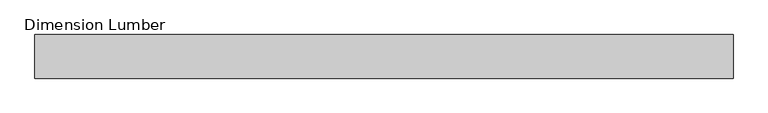
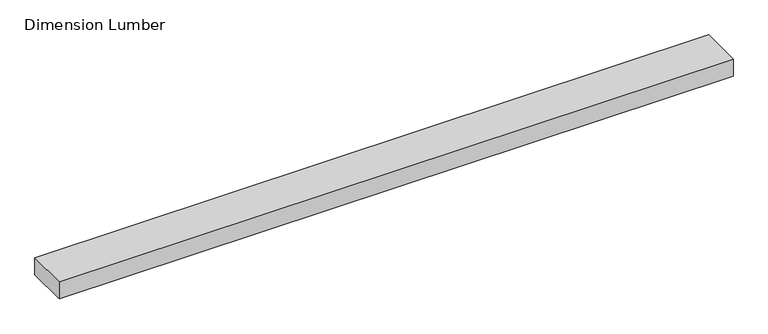
"""IFC4 building model written with IfcOpenShell, lengths in millimetres: beam geometry, Dimension Lumber : Top Supporting Lumbers."""

import ifcopenshell
import ifcopenshell.guid

model = None  # the IFC model being written
_history = None  # IfcOwnerHistory: only IFC2X3 demands one
_inside = {}  # id of a spatial element -> (the spatial element, [elements in it])
_under = {}  # id of a project, library or spatial element -> (it, [spatial elements below it])
_declared = {}  # id of a project -> (the project, [libraries it declares])
_typed = {}  # id of a type object -> (the type object, [elements of that type])
_made_of = {}  # id of a material, layer set ... -> (it, [elements and type objects made of it])


def new_model(schema):
    """Start an empty IFC model of exactly this schema.

    Asked for "IFC4X3", IfcOpenShell would pick the latest addendum, in which some entities
    have other attributes; the version numbers below select the first issue.
    IFC2X3 requires an IfcOwnerHistory on every rooted entity: one is made here for all.
    """
    global model, _history
    if schema == "IFC4X3":
        model = ifcopenshell.file(schema_version=(4, 3, 0, 0))
    else:
        model = ifcopenshell.file(schema=schema)
    _inside.clear()
    _under.clear()
    _declared.clear()
    _typed.clear()
    _made_of.clear()
    _history = None
    if model.schema == "IFC2X3":
        org = make("IfcOrganization", Name="unknown")
        user = make(
            "IfcPersonAndOrganization",
            ThePerson=make("IfcPerson", FamilyName="unknown"),
            TheOrganization=org,
        )
        app = make(
            "IfcApplication",
            ApplicationDeveloper=org,
            Version="unknown",
            ApplicationFullName="unknown",
            ApplicationIdentifier="unknown",
        )
        _history = make(
            "IfcOwnerHistory",
            OwningUser=user,
            OwningApplication=app,
            ChangeAction="ADDED",
            CreationDate=0,
        )
    return model


def make(cls, **values):
    """One entity of the class cls with the attributes given. An attribute that is None is left unset."""
    return model.create_entity(
        cls, **{name: value for name, value in values.items() if value is not None}
    )


def rooted(cls, **values):
    """An entity with a GlobalId (a new one), such as an element, a storey or a relation."""
    return make(cls, GlobalId=ifcopenshell.guid.new(), OwnerHistory=_history, **values)


def si_unit(unit_type, name, prefix=None):
    """IfcSIUnit, for example si_unit("LENGTHUNIT", "METRE", prefix="MILLI")."""
    return make("IfcSIUnit", UnitType=unit_type, Prefix=prefix, Name=name)


def assignment(units):
    """IfcUnitAssignment: the units of a project."""
    return None if units is None else make("IfcUnitAssignment", Units=units)


def point(xyz):
    """IfcCartesianPoint."""
    return None if xyz is None else make("IfcCartesianPoint", Coordinates=xyz)


def direction(xyz):
    """IfcDirection."""
    return None if xyz is None else make("IfcDirection", DirectionRatios=xyz)


def frame(location, z_axis=None, x_axis=None):
    """IfcAxis2Placement3D, a coordinate frame: its origin and axes. An axis left out is left unset."""
    return make(
        "IfcAxis2Placement3D",
        Location=point(location),
        Axis=direction(z_axis),
        RefDirection=direction(x_axis),
    )


def origin():
    """The frame at (0, 0, 0) with its axes left unset."""
    return frame((0.0, 0.0, 0.0))


def place(relative_to, where):
    """IfcLocalPlacement: puts the frame where relative to a parent placement (None: the world)."""
    return make(
        "IfcLocalPlacement", PlacementRelTo=relative_to, RelativePlacement=where
    )


def context(
    kind, dimensions, precision=None, world=None, true_north=None, identifier=None
):
    """IfcGeometricRepresentationContext, for example the 3D "Model" context."""
    return make(
        "IfcGeometricRepresentationContext",
        ContextIdentifier=identifier,
        ContextType=kind,
        CoordinateSpaceDimension=dimensions,
        Precision=precision,
        WorldCoordinateSystem=world,
        TrueNorth=true_north,
    )


def project(units=None, contexts=None):
    """IfcProject with its units and contexts."""
    return rooted(
        "IfcProject",
        Name="project",
        RepresentationContexts=contexts,
        UnitsInContext=assignment(units),
    )


def spatial(cls, under=None, at=None, **own):
    """A site, building, storey or space (cls), placed at a placement, below another one or the project."""
    s = rooted(cls, ObjectPlacement=at, **own)
    if under is not None:
        _under.setdefault(under.id(), (under, []))[1].append(s)
    return s


def polyline(points):
    """IfcPolyline through the points."""
    return make("IfcPolyline", Points=[point(p) for p in points])


def outline(outer, holes=None, kind="AREA"):
    """IfcArbitraryClosedProfileDef: a profile drawn as a closed curve; with holes, ...WithVoids."""
    if holes is None:
        return make("IfcArbitraryClosedProfileDef", ProfileType=kind, OuterCurve=outer)
    return make(
        "IfcArbitraryProfileDefWithVoids",
        ProfileType=kind,
        OuterCurve=outer,
        InnerCurves=holes,
    )


def extrude(swept, where, along, depth):
    """IfcExtrudedAreaSolid: the profile swept, set in the frame where, extruded along a direction by depth."""
    return make(
        "IfcExtrudedAreaSolid",
        SweptArea=swept,
        Position=where,
        ExtrudedDirection=direction(along),
        Depth=depth,
    )


def shape(context_of_items, identifier, shape_type, items):
    """IfcShapeRepresentation: the items that make up one representation, for example the "Body"."""
    return make(
        "IfcShapeRepresentation",
        ContextOfItems=context_of_items,
        RepresentationIdentifier=identifier,
        RepresentationType=shape_type,
        Items=items,
    )


def source(mapping_origin, context_of_items, identifier, shape_type, items):
    """IfcRepresentationMap: a shape defined once, which mapped items show again and again."""
    return make(
        "IfcRepresentationMap",
        MappingOrigin=mapping_origin,
        MappedRepresentation=shape(context_of_items, identifier, shape_type, items),
    )


def transform(
    local_origin,
    x_axis=None,
    y_axis=None,
    z_axis=None,
    scale=None,
    scale2=None,
    scale3=None,
    uniform=True,
):
    """IfcCartesianTransformationOperator3D, or its non-uniform kind. x_axis, y_axis, z_axis: its Axis1, 2, 3."""
    if uniform:
        return make(
            "IfcCartesianTransformationOperator3D",
            Axis1=direction(x_axis),
            Axis2=direction(y_axis),
            LocalOrigin=point(local_origin),
            Scale=scale,
            Axis3=direction(z_axis),
        )
    return make(
        "IfcCartesianTransformationOperator3DnonUniform",
        Axis1=direction(x_axis),
        Axis2=direction(y_axis),
        LocalOrigin=point(local_origin),
        Scale=scale,
        Axis3=direction(z_axis),
        Scale2=scale2,
        Scale3=scale3,
    )


def mapped(mapping_source, mapping_target):
    """IfcMappedItem: shows the shape of a source again, moved by a transform."""
    return make(
        "IfcMappedItem", MappingSource=mapping_source, MappingTarget=mapping_target
    )


def made_of(thing, what):
    """Note that an element or type object is made of a material, layer set ...; save() writes the relation."""
    if what is not None:
        _made_of.setdefault(what.id(), (what, []))[1].append(thing)
    return thing


def element(
    cls,
    number,
    at=None,
    inside=None,
    cuts=None,
    type_object=None,
    material=None,
    context=None,
    identifier="Body",
    shape_type=None,
    held_by="IfcProductDefinitionShape",
    body=None,
    shapes=None,
    **own,
):
    """One element of the class cls, such as IfcWall. Its Tag is "e" and its number.

    at: its placement. inside: the storey or other place that contains it. cuts: it is an
    opening in that element (IfcRelVoidsElement). A single representation is given by context,
    identifier, shape_type and body (its items); several are given by shapes. held_by: the class
    of the entity that holds the representations. save() writes the other relations.
    """
    e = rooted(cls, Tag="e%d" % number, ObjectPlacement=at, **own)
    if body is not None:
        shapes = [shape(context, identifier, shape_type, body)]
    if shapes is not None:
        e.Representation = make(held_by, Representations=shapes)
    if inside is not None:
        _inside.setdefault(inside.id(), (inside, []))[1].append(e)
    if cuts is not None:
        rooted(
            "IfcRelVoidsElement", RelatingBuildingElement=cuts, RelatedOpeningElement=e
        )
    if type_object is not None:
        _typed.setdefault(type_object.id(), (type_object, []))[1].append(e)
    return made_of(e, material)


def aggregate(whole, parts):
    """IfcRelAggregates: a whole, such as a stair, and the parts it consists of."""
    return rooted("IfcRelAggregates", RelatingObject=whole, RelatedObjects=parts)


def save(model, path):
    """Write the relations noted so far, then the file.

    IfcRelAggregates (storeys below a building ...), IfcRelContainedInSpatialStructure (elements
    in a storey), IfcRelDefinesByType, IfcRelAssociatesMaterial and IfcRelDeclares: one each for
    every whole, place, type object, material and project.
    """
    for whole, parts in _under.values():
        aggregate(whole, parts)
    for where, things in _inside.values():
        rooted(
            "IfcRelContainedInSpatialStructure",
            RelatedElements=things,
            RelatingStructure=where,
        )
    for kind, things in _typed.values():
        rooted("IfcRelDefinesByType", RelatedObjects=things, RelatingType=kind)
    for what, things in _made_of.values():
        rooted("IfcRelAssociatesMaterial", RelatedObjects=things, RelatingMaterial=what)
    for by, libraries in _declared.values():
        rooted("IfcRelDeclares", RelatingContext=by, RelatedDefinitions=libraries)
    model.write(path)


def dimension_lumber_71d4a028(model_context):
    return source(origin(), model_context, "Body", "SweptSolid", [
        extrude(outline(polyline([(5096.66875, -44.45), (3674.26875, -44.45), (3674.26875, 44.45), (5096.66875, 44.45), (5096.66875, -44.45)])), frame((0.0, 0.0, -19.05), z_axis=(0.0, 0.0, 1.0), x_axis=(1.0, 0.0, 0.0)), (0.0, 0.0, 1.0), 38.1),
    ])


if __name__ == "__main__":
    model = new_model("IFC4")
    model_context = context("Model", 3, world=origin())
    ifc_project = project(units=[si_unit("LENGTHUNIT", "METRE", prefix="MILLI")], contexts=[model_context])
    site = spatial("IfcSite", under=ifc_project)
    building = spatial("IfcBuilding", under=site)
    placement = place(None, origin())
    dimension_lumber_shape = dimension_lumber_71d4a028(model_context)
    element("IfcBeam", 1, ObjectType="Dimension Lumber : Top Supporting Lumbers", at=placement, inside=building, context=model_context, shape_type="MappedRepresentation", body=[
        mapped(dimension_lumber_shape, transform((0.0, 0.0, 0.0), x_axis=(1.0, 0.0, 0.0), y_axis=(0.0, 1.0, 0.0), z_axis=(0.0, 0.0, 1.0))),
    ])
    save(model, "model.ifc")

# Revit data of these elements
# Type "Dimension Lumber : Top Supporting Lumbers"
#   Assembly Code = "B10"
#   A = 0.0364583 SF
#   Length [instance default] = 5' - 0"
#   b = 0' - 3 1/2"
#   d = 0' - 1 1/2"
#   Structural Material [instance default] = Softwood, Lumber
# Element 1 (IfcBeam, "Dimension Lumber : Top Supporting Lumbers")
#   Structural Material = Douglas Fir #2
#   Materials on its faces: "Douglas Fir #2"
# Materials
#   "Softwood, Lumber": class "Wood", colour RGB 223 192 134, transparency 0, Description = "Pinus Echinata", Cost = 0
#   "Douglas Fir #2": class "Wood", colour RGB 223 192 134, transparency 0, Description = "Pinus Echinata", Cost = 0
